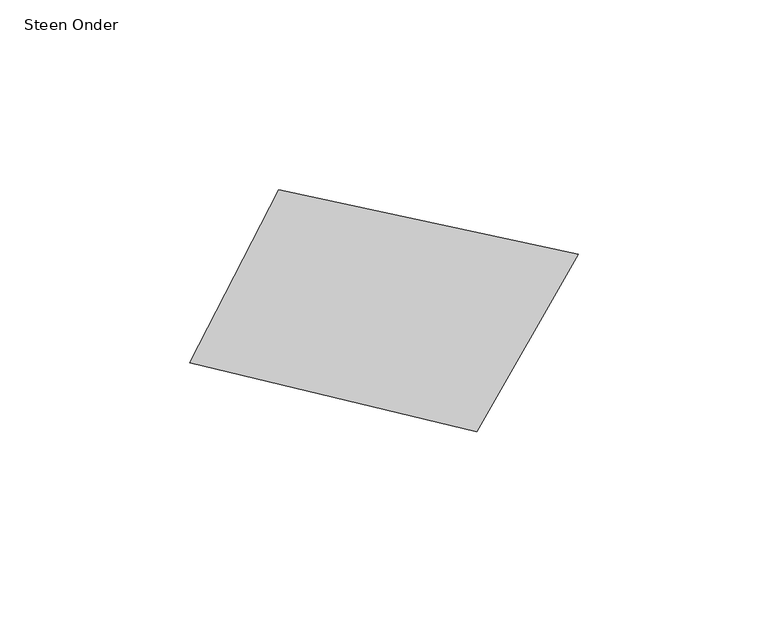
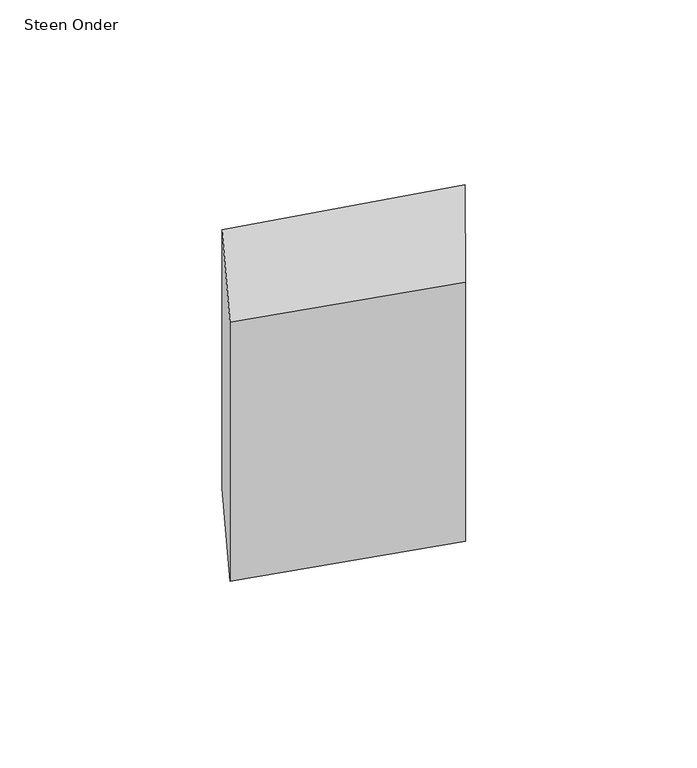
"""IFC4 building model written with IfcOpenShell, lengths in millimetres: proxy geometry, 00_GMA_steen_versie_4 : Steen Onder."""

from ifc_helpers import new_model, si_unit, frame, origin, place, context, project, spatial, polyline, outline, extrude, source, transform, mapped, element, save


def steen_onder_94586070(model_context):
    return source(origin(), model_context, "Body", "SweptSolid", [
        extrude(outline(polyline([(140.190891, 56.2230366), (113.4122173, 9.4519213), (37.8851218, 27.5806454), (61.3466084, 73.1941863), (140.190891, 56.2230366)])), frame((0.0, 0.0, -100.0), z_axis=(0.0, 0.0, 1.0), x_axis=(1.0, 0.0, 0.0)), (0.0, 0.0, 1.0), 100.0),
    ])


if __name__ == "__main__":
    model = new_model("IFC4")
    model_context = context("Model", 3, world=origin())
    ifc_project = project(units=[si_unit("LENGTHUNIT", "METRE", prefix="MILLI")], contexts=[model_context])
    site = spatial("IfcSite", under=ifc_project)
    building = spatial("IfcBuilding", under=site)
    placement = place(None, origin())
    steen_onder_shape = steen_onder_94586070(model_context)
    element("IfcBuildingElementProxy", 1, Name="00_GMA_steen_versie_4 : Steen Onder", ObjectType="00_GMA_steen_versie_4 : Steen Onder", at=placement, inside=building, context=model_context, shape_type="MappedRepresentation", body=[
        mapped(steen_onder_shape, transform((0.0, 0.0, 0.0), x_axis=(1.0, 0.0, 0.0), y_axis=(0.0, 1.0, 0.0), z_axis=(0.0, 0.0, 1.0))),
    ])
    save(model, "model.ifc")

# Revit data of these elements
# Type "00_GMA_steen_versie_4 : Steen Onder"
#   StootVoegHalfBoven [instance default] = 5 mm
#   StootVoegHalf [instance default] = 5 mm
#   StootVoegBreedteOnder = 10 mm
#   StootVoegBreedteBoven = 10 mm
#   Steendikte = 100 mm
#   LintVoegOnderHalf = 0 mm
#   LintVoegOnder = 0 mm
#   LintVoegBovenHalf = 5 mm
#   LintVoegBoven = 10 mm
#   materiaal = none
#   MateriaalVoeg = none
#   Default Elevation = 0
